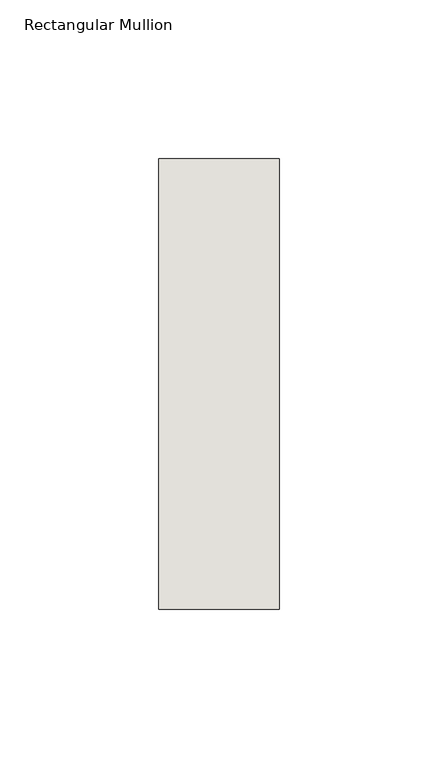
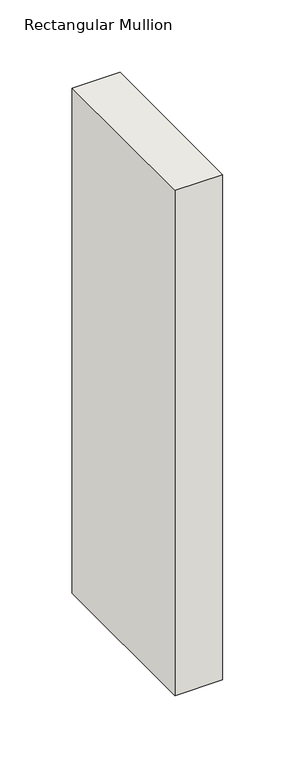
"""IFC4 building model written with IfcOpenShell, lengths in millimetres: wall geometry, Rectangular Mullion : NLRS_21_CWM_hsb-regel 38x142_gen_rsf."""

from ifc_helpers import new_model, si_unit, frame, origin, place, context, project, spatial, polyline, outline, extrude, source, transform, mapped, element, save


def rectangular_mullion_4d4fc8f4(model_context):
    return source(origin(), model_context, "Body", "SweptSolid", [
        extrude(outline(polyline([(0.0, -71.0), (-38.0, -71.0), (-38.0, 71.0), (0.0, 71.0), (0.0, -71.0)])), frame((0.0, 0.0, -426.0), z_axis=(0.0, 0.0, 1.0), x_axis=(1.0, 0.0, 0.0)), (0.0, 0.0, 1.0), 426.0),
    ])


if __name__ == "__main__":
    model = new_model("IFC4")
    model_context = context("Model", 3, world=origin())
    ifc_project = project(units=[si_unit("LENGTHUNIT", "METRE", prefix="MILLI")], contexts=[model_context])
    site = spatial("IfcSite", under=ifc_project)
    building = spatial("IfcBuilding", under=site)
    placement = place(None, origin())
    rectangular_mullion_shape = rectangular_mullion_4d4fc8f4(model_context)
    element("IfcWall", 1, ObjectType="Rectangular Mullion : NLRS_21_CWM_hsb-regel 38x142_gen_rsf", at=placement, inside=building, context=model_context, shape_type="MappedRepresentation", body=[
        mapped(rectangular_mullion_shape, transform((0.0, 0.0, 0.0), x_axis=(1.0, 0.0, 0.0), y_axis=(0.0, 1.0, 0.0), z_axis=(0.0, 0.0, 1.0))),
    ])
    save(model, "model.ifc")

# Revit data of these elements
# Type "Rectangular Mullion : NLRS_21_CWM_hsb-regel 38x142_gen_rsf"
#   Type IfcGUID = "07M7mRoiH1CR8m_RSKIwpF"
#   Assembly Code = "21.10"
#   IfcExportAs = "IfcWall"
#   built-in parameter 1007322 = 0.465879 (stored number, unit not read)
#   built-in parameter 1007321 = 0.062336 (stored number, unit not read)
#   built-in parameter 1007320 = 0.062336 (stored number, unit not read)
# Element 1 (IfcWall, "Rectangular Mullion : NLRS_21_CWM_hsb-regel 38x142_gen_rsf")
#   Materials on its faces: "NLRS_i2_hout naaldhout vuren_gen_rsf"
# Materials
#   "NLRS_i2_hout naaldhout vuren_gen_rsf": class "I - Hout", colour RGB 234 199 147, transparency 0, Keynote = "i2", Manufacturer = "Revit Standards Foundation", URL = "www.revitstandards.org", Description = "hout vuren", Cost = 0
